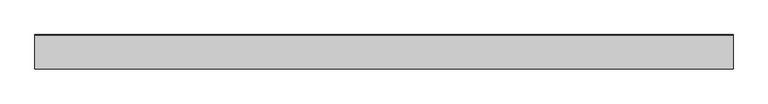
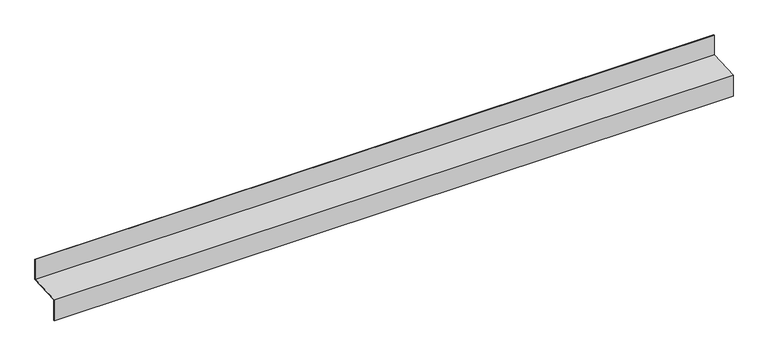
"""IFC4 building model written with IfcOpenShell, lengths in millimetres: proxy geometry, Generic Models 7:Generic Models 1:5:Generic Models 1:5 : Generic Models 7:Generic Models 1:337419:4 : Generic Models 7:Generic Models 1:5:Generic Models 1:5 : Generic Models 7:Generic Models 1:337419:311462."""

from ifc_helpers import new_model, si_unit, frame, origin, place, context, project, spatial, polyline, outline, extrude, source, transform, mapped, element, save


def generic_models_9e5cb043(model_context):
    return source(origin(), model_context, "Body", "SweptSolid", [
        extrude(outline(polyline([(-579143.6477614, -76.436279), (-579145.2352614, -76.436279), (-579145.2352614, 4.0632001), (-579026.1727614, 9.0241376), (-579026.1727614, 84.3642418), (-579024.5852614, 84.3642418), (-579024.5852614, 7.501406), (-579143.6477614, 2.5404685), (-579143.6477614, -76.436279)])), frame((570452.6367239, 0.0, 0.0), z_axis=(1.0, 0.0, 0.0), x_axis=(0.0, 1.0, 0.0)), (0.0, 0.0, 1.0), 2444.75),
    ])


if __name__ == "__main__":
    model = new_model("IFC4")
    model_context = context("Model", 3, world=origin())
    ifc_project = project(units=[si_unit("LENGTHUNIT", "METRE", prefix="MILLI")], contexts=[model_context])
    site = spatial("IfcSite", under=ifc_project)
    building = spatial("IfcBuilding", under=site)
    placement = place(None, origin())
    generic_models_shape = generic_models_9e5cb043(model_context)
    element("IfcBuildingElementProxy", 1, Name="Generic Models 7:Generic Models 1:5:Generic Models 1:5 : Generic Models 7:Generic Models 1:337419:4 : Generic Models 7:Generic Models 1:5:Generic Models 1:5 : Generic Models 7:Generic Models 1:337419:311462", ObjectType="Generic Models 7:Generic Models 1:5:Generic Models 1:5 : Generic Models 7:Generic Models 1:337419:4 : Generic Models 7:Generic Models 1:5:Generic Models 1:5 : Generic Models 7:Generic Models 1:337419:311462", at=placement, inside=building, context=model_context, shape_type="MappedRepresentation", body=[
        mapped(generic_models_shape, transform((0.0, 0.0, 0.0), x_axis=(1.0, 0.0, 0.0), y_axis=(0.0, 1.0, 0.0), z_axis=(0.0, 0.0, 1.0))),
    ])
    save(model, "model.ifc")

# Revit data of these elements
# Type "Generic Models 7:Generic Models 1:5:Generic Models 1:5 : Generic Models 7:Generic Models 1:337419:4 : Generic Models 7:Generic Models 1:5:Generic Models 1:5 : Generic Models 7:Generic Models 1:337419:311462"
#   NameOverride = "Generic Models 7:Generic Models 1:5:Generic Models 1:5 : Generic Models 7:Generic Models 1:337419:311462"
#   ObjectTypeOverride = "Generic Models 1:5 : Generic Models 7:Generic Models 1:337419"
#   Reference = "Generic Models 1"
#   Tag = "311462"
# Element 1 (IfcBuildingElementProxy, "Generic Models 7:Generic Models 1:5:Generic Models 1:5 : Generic Models 7:Generic Models 1:337419:4 : Generic Models 7:Generic Models 1:5:Generic Models 1:5 : Generic Models 7:Generic Models 1:337419:311462")
#   Materials on its faces: "BRAKE METAL FLASHING WITH BACK & END DAMS"
# Materials
#   "BRAKE METAL FLASHING WITH BACK & END DAMS": class "Unassigned", colour RGB 182 182 182, transparency 0, Cost = 0
